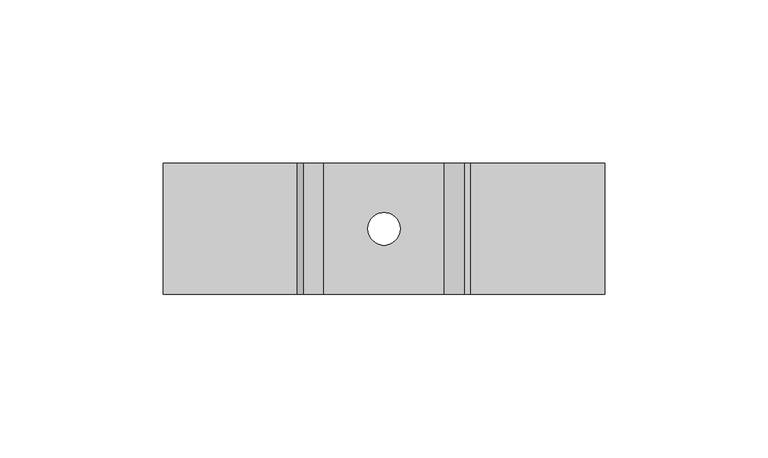
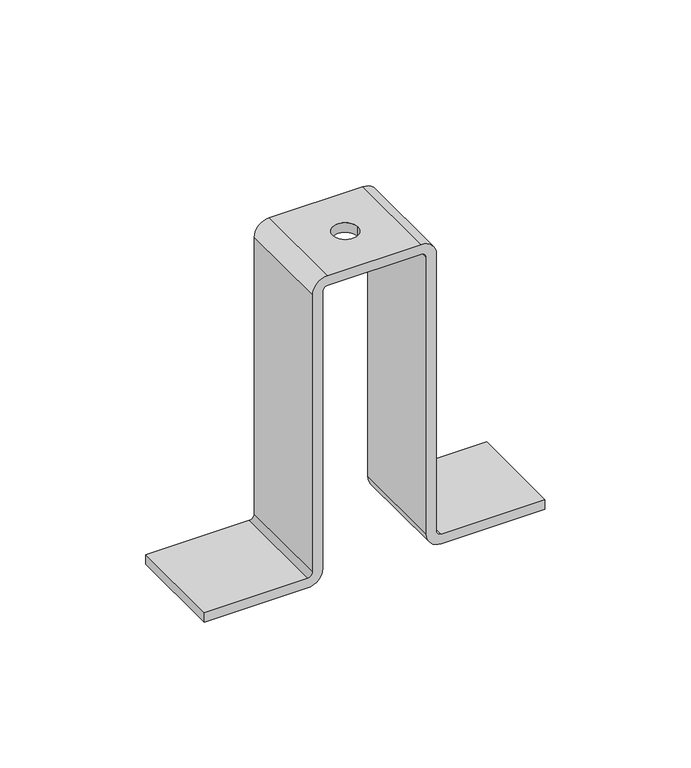
"""IFC4 building model written with IfcOpenShell, lengths in millimetres: proxy geometry, ▶ TN_Скоба соединительная (сборка тип 1) : ▶ TN_Скоба соединительная (сборка тип 1)."""

from ifc_helpers import new_model, si_unit, frame, origin, place, context, project, spatial, polyline, circle_curve, source, transform, mapped, element, save
from ifc_brep_helpers import plane_surface, cylinder_surface, revolved_surface, advanced_brep


def generic_models_70dbd3d5(model_context):
    return source(origin(), model_context, "Body", "AdvancedBrep", [
        advanced_brep(
        [(-5.0, 0.0, 124.0), (-5.0, 0.0, 128.0), (5.0, 0.0, 128.0), (5.0, 0.0, 124.0), (-26.5, -20.0, 0.0), (-20.5, -20.0, 6.0), (-20.5, -20.0, 122.0), (-18.5, -20.0, 124.0), (18.5, -20.0, 124.0), (20.5, -20.0, 122.0), (20.5, -20.0, 6.0), (26.5, -20.0, 0.0), (67.5, -20.0, 0.0), (67.5, -20.0, 4.0), (26.5, -20.0, 4.0), (24.5, -20.0, 6.0), (24.5, -20.0, 122.0), (18.5, -20.0, 128.0), (-18.5, -20.0, 128.0), (-24.5, -20.0, 122.0), (-24.5, -20.0, 6.0), (-26.5, -20.0, 4.0), (-67.5, -20.0, 4.0), (-67.5, -20.0, 0.0), (-26.5, 20.0, 0.0), (-67.5, 20.0, 0.0), (-67.5, 20.0, 4.0), (-26.5, 20.0, 4.0), (-24.5, 20.0, 6.0), (-24.5, 20.0, 122.0), (-18.5, 20.0, 128.0), (18.5, 20.0, 128.0), (24.5, 20.0, 122.0), (24.5, 20.0, 6.0), (26.5, 20.0, 4.0), (67.5, 20.0, 4.0), (67.5, 20.0, 0.0), (26.5, 20.0, 0.0), (20.5, 20.0, 6.0), (20.5, 20.0, 122.0), (18.5, 20.0, 124.0), (-18.5, 20.0, 124.0), (-20.5, 20.0, 122.0), (-20.5, 20.0, 6.0)],
        [
            (0, 1),
            (1, 2, circle_curve(frame((0.0, 0.0, 128.0), z_axis=(0.0, 0.0, 1.0), x_axis=(1.0, 0.0, 0.0)), 5.0)),
            (2, 3),
            (3, 0, circle_curve(frame((0.0, 0.0, 124.0), z_axis=(0.0, 0.0, -1.0), x_axis=(1.0, 0.0, 0.0)), 5.0)),
            (0, 3, circle_curve(frame((0.0, 0.0, 124.0), z_axis=(0.0, 0.0, -1.0), x_axis=(1.0, 0.0, 0.0)), 5.0)),
            (2, 1, circle_curve(frame((0.0, 0.0, 128.0), z_axis=(0.0, 0.0, 1.0), x_axis=(1.0, 0.0, 0.0)), 5.0)),
            (4, 5, circle_curve(frame((-26.5, -20.0, 6.0), z_axis=(0.0, -1.0, 0.0), x_axis=(0.0, 0.0, -1.0)), 6.0)),
            (5, 6),
            (6, 7, circle_curve(frame((-18.5, -20.0, 122.0), z_axis=(0.0, 1.0, 0.0), x_axis=(0.0, 0.0, -1.0)), 2.0)),
            (7, 8),
            (8, 9, circle_curve(frame((18.5, -20.0, 122.0), z_axis=(0.0, 1.0, 0.0), x_axis=(0.0, 0.0, -1.0)), 2.0)),
            (9, 10),
            (10, 11, circle_curve(frame((26.5, -20.0, 6.0), z_axis=(0.0, -1.0, 0.0), x_axis=(0.0, 0.0, -1.0)), 6.0)),
            (11, 12),
            (12, 13),
            (13, 14),
            (14, 15, circle_curve(frame((26.5, -20.0, 6.0), z_axis=(0.0, 1.0, 0.0), x_axis=(0.0, 0.0, -1.0)), 2.0)),
            (15, 16),
            (16, 17, circle_curve(frame((18.5, -20.0, 122.0), z_axis=(0.0, -1.0, 0.0), x_axis=(0.0, 0.0, -1.0)), 6.0)),
            (17, 18),
            (18, 19, circle_curve(frame((-18.5, -20.0, 122.0), z_axis=(0.0, -1.0, 0.0), x_axis=(0.0, 0.0, -1.0)), 6.0)),
            (19, 20),
            (20, 21, circle_curve(frame((-26.5, -20.0, 6.0), z_axis=(0.0, 1.0, 0.0), x_axis=(0.0, 0.0, -1.0)), 2.0)),
            (21, 22),
            (22, 23),
            (23, 4),
            (24, 25),
            (25, 26),
            (26, 27),
            (27, 28, circle_curve(frame((-26.5, 20.0, 6.0), z_axis=(0.0, -1.0, 0.0), x_axis=(0.0, 0.0, -1.0)), 2.0)),
            (28, 29),
            (29, 30, circle_curve(frame((-18.5, 20.0, 122.0), z_axis=(0.0, 1.0, 0.0), x_axis=(0.0, 0.0, -1.0)), 6.0)),
            (30, 31),
            (31, 32, circle_curve(frame((18.5, 20.0, 122.0), z_axis=(0.0, 1.0, 0.0), x_axis=(0.0, 0.0, -1.0)), 6.0)),
            (32, 33),
            (33, 34, circle_curve(frame((26.5, 20.0, 6.0), z_axis=(0.0, -1.0, 0.0), x_axis=(0.0, 0.0, -1.0)), 2.0)),
            (34, 35),
            (35, 36),
            (36, 37),
            (37, 38, circle_curve(frame((26.5, 20.0, 6.0), z_axis=(0.0, 1.0, 0.0), x_axis=(0.0, 0.0, -1.0)), 6.0)),
            (38, 39),
            (39, 40, circle_curve(frame((18.5, 20.0, 122.0), z_axis=(0.0, -1.0, 0.0), x_axis=(0.0, 0.0, -1.0)), 2.0)),
            (40, 41),
            (41, 42, circle_curve(frame((-18.5, 20.0, 122.0), z_axis=(0.0, -1.0, 0.0), x_axis=(0.0, 0.0, -1.0)), 2.0)),
            (42, 43),
            (43, 24, circle_curve(frame((-26.5, 20.0, 6.0), z_axis=(0.0, 1.0, 0.0), x_axis=(0.0, 0.0, -1.0)), 6.0)),
            (4, 24),
            (43, 5),
            (42, 6),
            (41, 7),
            (40, 8),
            (39, 9),
            (38, 10),
            (37, 11),
            (36, 12),
            (35, 13),
            (34, 14),
            (33, 15),
            (32, 16),
            (31, 17),
            (30, 18),
            (29, 19),
            (28, 20),
            (27, 21),
            (26, 22),
            (25, 23),
        ],
        [
            revolved_surface(polyline([(5.0, 0.0, 128.0), (5.0, 0.0, 124.0)]), (0.0, 0.0, 35.2036226), (0.0, 0.0, 1.0)),
            plane_surface(frame((0.0, -20.0, 0.0), z_axis=(0.0, -1.0, 0.0), x_axis=(0.0, 0.0, 1.0))),
            plane_surface(frame((0.0, 20.0, 0.0), z_axis=(0.0, 1.0, 0.0), x_axis=(0.0, 0.0, 1.0))),
            cylinder_surface(frame((-26.5, -20.0, 6.0), z_axis=(0.0, -1.0, 0.0), x_axis=(0.0, 0.0, -1.0)), 6.0),
            plane_surface(frame((-20.5, -20.0, 6.0), z_axis=(1.0, 0.0, 0.0), x_axis=(0.0, 1.0, 0.0))),
            revolved_surface(polyline([(-18.5, 20.0, 120.0), (-18.5, -20.0, 120.0)]), (-18.5, -20.0, 122.0), (0.0, 1.0, 0.0)),
            plane_surface(frame((-18.5, -20.0, 124.0), z_axis=(0.0, 0.0, -1.0), x_axis=(0.0, 1.0, 0.0))),
            revolved_surface(polyline([(18.5, 20.0, 120.0), (18.5, -20.0, 120.0)]), (18.5, -20.0, 122.0), (0.0, 1.0, 0.0)),
            plane_surface(frame((20.5, -20.0, 122.0), z_axis=(-1.0, 0.0, 0.0), x_axis=(0.0, 1.0, 0.0))),
            cylinder_surface(frame((26.5, -20.0, 6.0), z_axis=(0.0, -1.0, 0.0), x_axis=(0.0, 0.0, -1.0)), 6.0),
            plane_surface(frame((26.5, -20.0, 0.0), z_axis=(0.0, 0.0, -1.0), x_axis=(0.0, 1.0, 0.0))),
            plane_surface(frame((67.5, -20.0, 0.0), z_axis=(1.0, 0.0, 0.0), x_axis=(0.0, 1.0, 0.0))),
            plane_surface(frame((67.5, -20.0, 4.0), z_axis=(0.0, 0.0, 1.0), x_axis=(0.0, 1.0, 0.0))),
            revolved_surface(polyline([(26.5, 20.0, 4.0), (26.5, -20.0, 4.0)]), (26.5, -20.0, 6.0), (0.0, 1.0, 0.0)),
            plane_surface(frame((24.5, -20.0, 6.0), z_axis=(1.0, 0.0, 0.0), x_axis=(0.0, 1.0, 0.0))),
            cylinder_surface(frame((18.5, -20.0, 122.0), z_axis=(0.0, -1.0, 0.0), x_axis=(0.0, 0.0, -1.0)), 6.0),
            plane_surface(frame((18.5, -20.0, 128.0), z_axis=(0.0, 0.0, 1.0), x_axis=(0.0, 1.0, 0.0))),
            cylinder_surface(frame((-18.5, -20.0, 122.0), z_axis=(0.0, -1.0, 0.0), x_axis=(0.0, 0.0, -1.0)), 6.0),
            plane_surface(frame((-24.5, -20.0, 122.0), z_axis=(-1.0, 0.0, 0.0), x_axis=(0.0, 1.0, 0.0))),
            revolved_surface(polyline([(-26.5, 20.0, 4.0), (-26.5, -20.0, 4.0)]), (-26.5, -20.0, 6.0), (0.0, 1.0, 0.0)),
            plane_surface(frame((-26.5, -20.0, 4.0), z_axis=(0.0, 0.0, 1.0), x_axis=(0.0, 1.0, 0.0))),
            plane_surface(frame((-67.5, -20.0, 4.0), z_axis=(-1.0, 0.0, 0.0), x_axis=(0.0, 1.0, 0.0))),
            plane_surface(frame((-67.5, -20.0, 0.0), z_axis=(0.0, 0.0, -1.0), x_axis=(0.0, 1.0, 0.0))),
        ],
        [
            (0, [[1, 2, 3, 4]]),
            (0, [[-1, 5, -3, 6]]),
            (1, [[7, 8, 9, 10, 11, 12, 13, 14, 15, 16, 17, 18, 19, 20, 21, 22, 23, 24, 25, 26]]),
            (2, [[27, 28, 29, 30, 31, 32, 33, 34, 35, 36, 37, 38, 39, 40, 41, 42, 43, 44, 45, 46]]),
            (3, [[-7, 47, -46, 48]]),
            (4, [[-8, -48, -45, 49]]),
            (5, [[-9, -49, -44, 50]]),
            (6, [[-10, -50, -43, 51], [-4, -5]]),
            (7, [[-11, -51, -42, 52]]),
            (8, [[-12, -52, -41, 53]]),
            (9, [[-13, -53, -40, 54]]),
            (10, [[-14, -54, -39, 55]]),
            (11, [[-15, -55, -38, 56]]),
            (12, [[-16, -56, -37, 57]]),
            (13, [[-17, -57, -36, 58]]),
            (14, [[-18, -58, -35, 59]]),
            (15, [[-19, -59, -34, 60]]),
            (16, [[-20, -60, -33, 61], [-2, -6]]),
            (17, [[-21, -61, -32, 62]]),
            (18, [[-22, -62, -31, 63]]),
            (19, [[-23, -63, -30, 64]]),
            (20, [[-24, -64, -29, 65]]),
            (21, [[-25, -65, -28, 66]]),
            (22, [[-26, -66, -27, -47]]),
        ],
    ),
    ])


if __name__ == "__main__":
    model = new_model("IFC4")
    model_context = context("Model", 3, world=origin())
    ifc_project = project(units=[si_unit("LENGTHUNIT", "METRE", prefix="MILLI")], contexts=[model_context])
    site = spatial("IfcSite", under=ifc_project)
    building = spatial("IfcBuilding", under=site)
    placement = place(None, origin())
    generic_models_shape = generic_models_70dbd3d5(model_context)
    element("IfcBuildingElementProxy", 1, Name="▶ TN_Скоба соединительная (сборка тип 1) : ▶ TN_Скоба соединительная (сборка тип 1)", ObjectType="▶ TN_Скоба соединительная (сборка тип 1) : ▶ TN_Скоба соединительная (сборка тип 1)", at=placement, inside=building, context=model_context, shape_type="MappedRepresentation", body=[
        mapped(generic_models_shape, transform((0.0, 0.0, 0.0), x_axis=(1.0, 0.0, 0.0), y_axis=(0.0, 1.0, 0.0), z_axis=(0.0, 0.0, 1.0))),
    ])
    save(model, "model.ifc")

# Revit data of these elements
# Type "▶ TN_Скоба соединительная (сборка тип 1) : ▶ TN_Скоба соединительная (сборка тип 1)"
#   Description = "Cоединительный элемент для монтажа рам, стеллажей, каркасов для легких и средних систем. Обеспечивает устойчивое поперечное (крестовое) соединение профилей. Наиболее эффективно использования скобы, как соединителя для создания пространственных силовых, опорных каркасов и решеток. Возможность реализации крепления профиля к бетонному основанию."
#   Manufacturer = "ТехноНИКОЛЬ"
#   Model = "Комплектующие к опорам"
#   URL = "https://nav.tn.ru/knowledge-base/polimernye-membrany/opory-pod-oborudovanie-na-ploskoy-krovle/?sphrase_id=266812"
#   ADSK_Обозначение = "ТехноНИКОЛЬ"
#   ADSK_Наименование краткое [instance default] = "С41х124 4F3"
#   ADSK_Наименование [instance default] = "Скоба соединительная 41х124 4F3"
#   ADSK_Масса_Текст = ""
#   ADSK_Марка [instance default] = "С41х124 4F3"
#   ADSK_Код изделия [instance default] = "690885"
#   ADSK_Завод-изготовитель = "ТехноНИКОЛЬ"
#   ADSK_Единица измерения = "шт."
#   ADSK_Группирование = "Комплектующие к опорам"
#   ADSK_URL страницы изделия = "https://nav.tn.ru/knowledge-base/polimernye-membrany/opory-pod-oborudovanie-na-ploskoy-krovle/?sphrase_id=266812"
#   ADSK_URL документации изделия = ""
#   Высота крепежа [instance default] = 84 mm
#   ADSK_Количество = 1
#   Скоба соединительная 41х62 4F3 [instance default] = no
#   Скоба соединительная 41х41 4F5 [instance default] = no
#   Скоба соединительная 41х124 4F3 [instance default] = yes
#   ADSK_Материал = TN_СтальГальванизированная_Серый
#   Default Elevation = 0
# Element 1 (IfcBuildingElementProxy, "▶ TN_Скоба соединительная (сборка тип 1) : ▶ TN_Скоба соединительная (сборка тип 1)")
#   Materials on its faces: "TN_СтальГальванизированная_Серый"
# Materials
#   "TN_СтальГальванизированная_Серый": class "Типовые", colour RGB 206 210 213, transparency 0, Cost = 0
